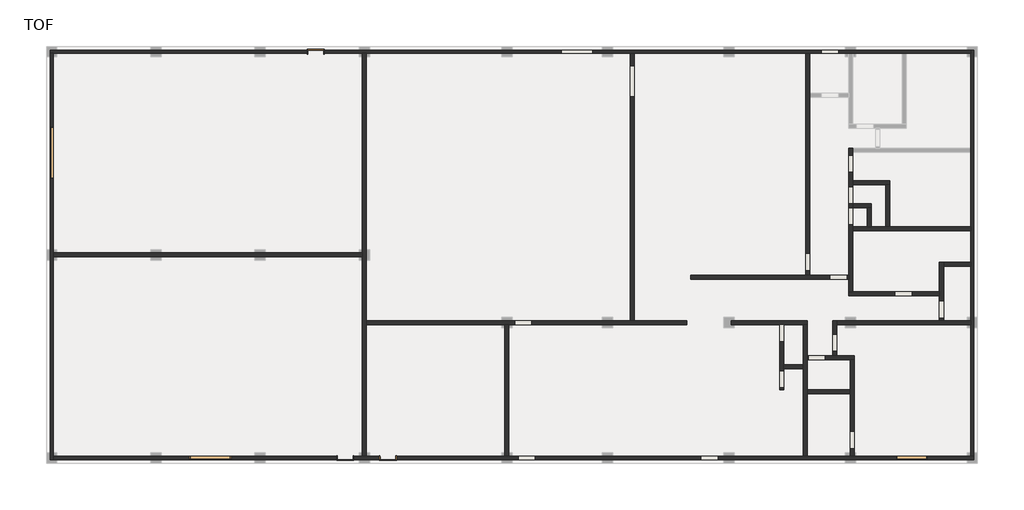
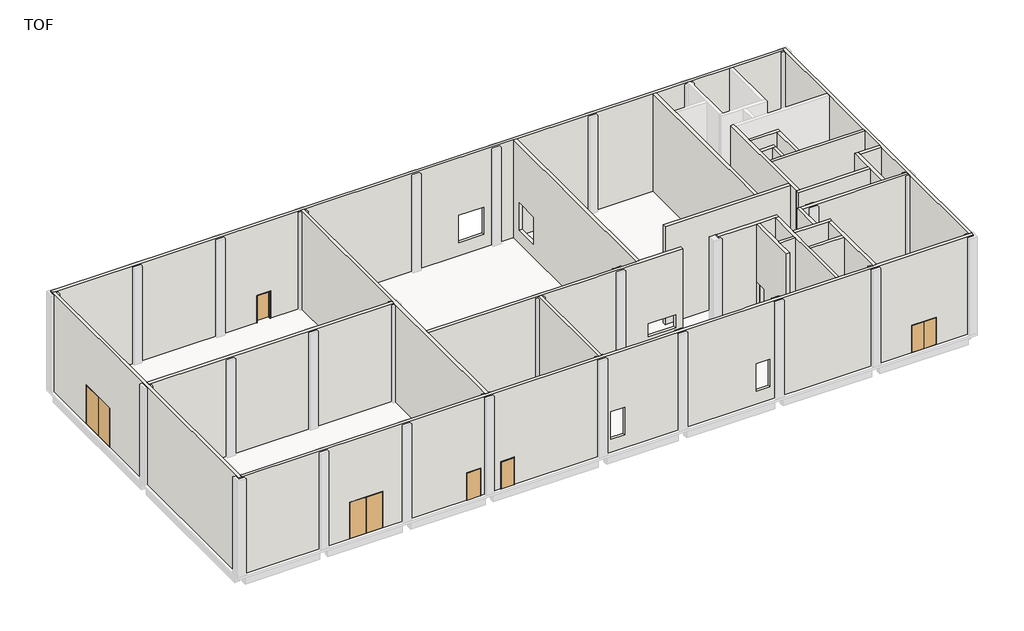
# One storey, part 1 of 2: 29 walls, 6 doors.
"""IFC4 building model written with IfcOpenShell, lengths in millimetres."""

import ifcopenshell
import ifcopenshell.guid

model = None  # the IFC model being written
_history = None  # IfcOwnerHistory: only IFC2X3 demands one
_inside = {}  # id of a spatial element -> (the spatial element, [elements in it])
_under = {}  # id of a project, library or spatial element -> (it, [spatial elements below it])
_declared = {}  # id of a project -> (the project, [libraries it declares])
_typed = {}  # id of a type object -> (the type object, [elements of that type])
_made_of = {}  # id of a material, layer set ... -> (it, [elements and type objects made of it])


def new_model(schema):
    """Start an empty IFC model of exactly this schema.

    Asked for "IFC4X3", IfcOpenShell would pick the latest addendum, in which some entities
    have other attributes; the version numbers below select the first issue.
    IFC2X3 requires an IfcOwnerHistory on every rooted entity: one is made here for all.
    """
    global model, _history
    if schema == "IFC4X3":
        model = ifcopenshell.file(schema_version=(4, 3, 0, 0))
    else:
        model = ifcopenshell.file(schema=schema)
    _inside.clear()
    _under.clear()
    _declared.clear()
    _typed.clear()
    _made_of.clear()
    _history = None
    if model.schema == "IFC2X3":
        org = make("IfcOrganization", Name="unknown")
        user = make(
            "IfcPersonAndOrganization",
            ThePerson=make("IfcPerson", FamilyName="unknown"),
            TheOrganization=org,
        )
        app = make(
            "IfcApplication",
            ApplicationDeveloper=org,
            Version="unknown",
            ApplicationFullName="unknown",
            ApplicationIdentifier="unknown",
        )
        _history = make(
            "IfcOwnerHistory",
            OwningUser=user,
            OwningApplication=app,
            ChangeAction="ADDED",
            CreationDate=0,
        )
    return model


def make(cls, **values):
    """One entity of the class cls with the attributes given. An attribute that is None is left unset."""
    return model.create_entity(
        cls, **{name: value for name, value in values.items() if value is not None}
    )


def rooted(cls, **values):
    """An entity with a GlobalId (a new one), such as an element, a storey or a relation."""
    return make(cls, GlobalId=ifcopenshell.guid.new(), OwnerHistory=_history, **values)


def si_unit(unit_type, name, prefix=None):
    """IfcSIUnit, for example si_unit("LENGTHUNIT", "METRE", prefix="MILLI")."""
    return make("IfcSIUnit", UnitType=unit_type, Prefix=prefix, Name=name)


def assignment(units):
    """IfcUnitAssignment: the units of a project."""
    return None if units is None else make("IfcUnitAssignment", Units=units)


def point(xyz):
    """IfcCartesianPoint."""
    return None if xyz is None else make("IfcCartesianPoint", Coordinates=xyz)


def direction(xyz):
    """IfcDirection."""
    return None if xyz is None else make("IfcDirection", DirectionRatios=xyz)


def frame(location, z_axis=None, x_axis=None):
    """IfcAxis2Placement3D, a coordinate frame: its origin and axes. An axis left out is left unset."""
    return make(
        "IfcAxis2Placement3D",
        Location=point(location),
        Axis=direction(z_axis),
        RefDirection=direction(x_axis),
    )


def origin():
    """The frame at (0, 0, 0) with its axes left unset."""
    return frame((0.0, 0.0, 0.0))


def origin_with_axes():
    """The frame at (0, 0, 0) with the z axis (0, 0, 1) and the x axis (1, 0, 0) written out."""
    return frame((0.0, 0.0, 0.0), z_axis=(0.0, 0.0, 1.0), x_axis=(1.0, 0.0, 0.0))


def place(relative_to, where):
    """IfcLocalPlacement: puts the frame where relative to a parent placement (None: the world)."""
    return make(
        "IfcLocalPlacement", PlacementRelTo=relative_to, RelativePlacement=where
    )


def context(
    kind, dimensions, precision=None, world=None, true_north=None, identifier=None
):
    """IfcGeometricRepresentationContext, for example the 3D "Model" context."""
    return make(
        "IfcGeometricRepresentationContext",
        ContextIdentifier=identifier,
        ContextType=kind,
        CoordinateSpaceDimension=dimensions,
        Precision=precision,
        WorldCoordinateSystem=world,
        TrueNorth=true_north,
    )


def project(units=None, contexts=None):
    """IfcProject with its units and contexts."""
    return rooted(
        "IfcProject",
        Name="project",
        RepresentationContexts=contexts,
        UnitsInContext=assignment(units),
    )


def spatial(cls, under=None, at=None, **own):
    """A site, building, storey or space (cls), placed at a placement, below another one or the project."""
    s = rooted(cls, ObjectPlacement=at, **own)
    if under is not None:
        _under.setdefault(under.id(), (under, []))[1].append(s)
    return s


def polyline(points):
    """IfcPolyline through the points."""
    return make("IfcPolyline", Points=[point(p) for p in points])


def outline(outer, holes=None, kind="AREA"):
    """IfcArbitraryClosedProfileDef: a profile drawn as a closed curve; with holes, ...WithVoids."""
    if holes is None:
        return make("IfcArbitraryClosedProfileDef", ProfileType=kind, OuterCurve=outer)
    return make(
        "IfcArbitraryProfileDefWithVoids",
        ProfileType=kind,
        OuterCurve=outer,
        InnerCurves=holes,
    )


def extrude(swept, where, along, depth):
    """IfcExtrudedAreaSolid: the profile swept, set in the frame where, extruded along a direction by depth."""
    return make(
        "IfcExtrudedAreaSolid",
        SweptArea=swept,
        Position=where,
        ExtrudedDirection=direction(along),
        Depth=depth,
    )


def faces_of(points, faces, orient=None, outer=None):
    """IfcFace entities. A face is a list of loops; a loop is a list of indices into points, from 0.

    orient and outer hold one flag for each loop. By default every Orientation is true, the
    first loop of a face is its IfcFaceOuterBound and the others are IfcFaceBound.
    """
    made = []
    for i, loops in enumerate(faces):
        bounds = []
        for j, loop in enumerate(loops):
            is_outer = j == 0 if outer is None else outer[i][j]
            bounds.append(
                make(
                    "IfcFaceOuterBound" if is_outer else "IfcFaceBound",
                    Bound=make("IfcPolyLoop", Polygon=[points[k] for k in loop]),
                    Orientation=True if orient is None else orient[i][j],
                )
            )
        made.append(make("IfcFace", Bounds=bounds))
    return made


def faceted_brep(points, faces, orient=None, outer=None, voids=None):
    """IfcFacetedBrep: a solid bounded by flat faces; with voids (closed shells), ...WithVoids."""
    shared = [point(p) for p in points]
    hull = make("IfcClosedShell", CfsFaces=faces_of(shared, faces, orient, outer))
    if voids is None:
        return make("IfcFacetedBrep", Outer=hull)
    return make(
        "IfcFacetedBrepWithVoids",
        Outer=hull,
        Voids=[
            make(cls, CfsFaces=faces_of(shared, fs, o, b)) for cls, fs, o, b in voids
        ],
    )


def shape(context_of_items, identifier, shape_type, items):
    """IfcShapeRepresentation: the items that make up one representation, for example the "Body"."""
    return make(
        "IfcShapeRepresentation",
        ContextOfItems=context_of_items,
        RepresentationIdentifier=identifier,
        RepresentationType=shape_type,
        Items=items,
    )


def source(mapping_origin, context_of_items, identifier, shape_type, items):
    """IfcRepresentationMap: a shape defined once, which mapped items show again and again."""
    return make(
        "IfcRepresentationMap",
        MappingOrigin=mapping_origin,
        MappedRepresentation=shape(context_of_items, identifier, shape_type, items),
    )


def transform(
    local_origin,
    x_axis=None,
    y_axis=None,
    z_axis=None,
    scale=None,
    scale2=None,
    scale3=None,
    uniform=True,
):
    """IfcCartesianTransformationOperator3D, or its non-uniform kind. x_axis, y_axis, z_axis: its Axis1, 2, 3."""
    if uniform:
        return make(
            "IfcCartesianTransformationOperator3D",
            Axis1=direction(x_axis),
            Axis2=direction(y_axis),
            LocalOrigin=point(local_origin),
            Scale=scale,
            Axis3=direction(z_axis),
        )
    return make(
        "IfcCartesianTransformationOperator3DnonUniform",
        Axis1=direction(x_axis),
        Axis2=direction(y_axis),
        LocalOrigin=point(local_origin),
        Scale=scale,
        Axis3=direction(z_axis),
        Scale2=scale2,
        Scale3=scale3,
    )


def mapped(mapping_source, mapping_target):
    """IfcMappedItem: shows the shape of a source again, moved by a transform."""
    return make(
        "IfcMappedItem", MappingSource=mapping_source, MappingTarget=mapping_target
    )


def made_of(thing, what):
    """Note that an element or type object is made of a material, layer set ...; save() writes the relation."""
    if what is not None:
        _made_of.setdefault(what.id(), (what, []))[1].append(thing)
    return thing


def element(
    cls,
    number,
    at=None,
    inside=None,
    cuts=None,
    type_object=None,
    material=None,
    context=None,
    identifier="Body",
    shape_type=None,
    held_by="IfcProductDefinitionShape",
    body=None,
    shapes=None,
    **own,
):
    """One element of the class cls, such as IfcWall. Its Tag is "e" and its number.

    at: its placement. inside: the storey or other place that contains it. cuts: it is an
    opening in that element (IfcRelVoidsElement). A single representation is given by context,
    identifier, shape_type and body (its items); several are given by shapes. held_by: the class
    of the entity that holds the representations. save() writes the other relations.
    """
    e = rooted(cls, Tag="e%d" % number, ObjectPlacement=at, **own)
    if body is not None:
        shapes = [shape(context, identifier, shape_type, body)]
    if shapes is not None:
        e.Representation = make(held_by, Representations=shapes)
    if inside is not None:
        _inside.setdefault(inside.id(), (inside, []))[1].append(e)
    if cuts is not None:
        rooted(
            "IfcRelVoidsElement", RelatingBuildingElement=cuts, RelatedOpeningElement=e
        )
    if type_object is not None:
        _typed.setdefault(type_object.id(), (type_object, []))[1].append(e)
    return made_of(e, material)


def aggregate(whole, parts):
    """IfcRelAggregates: a whole, such as a stair, and the parts it consists of."""
    return rooted("IfcRelAggregates", RelatingObject=whole, RelatedObjects=parts)


def save(model, path):
    """Write the relations noted so far, then the file.

    IfcRelAggregates (storeys below a building ...), IfcRelContainedInSpatialStructure (elements
    in a storey), IfcRelDefinesByType, IfcRelAssociatesMaterial and IfcRelDeclares: one each for
    every whole, place, type object, material and project.
    """
    for whole, parts in _under.values():
        aggregate(whole, parts)
    for where, things in _inside.values():
        rooted(
            "IfcRelContainedInSpatialStructure",
            RelatedElements=things,
            RelatingStructure=where,
        )
    for kind, things in _typed.values():
        rooted("IfcRelDefinesByType", RelatedObjects=things, RelatingType=kind)
    for what, things in _made_of.values():
        rooted("IfcRelAssociatesMaterial", RelatedObjects=things, RelatingMaterial=what)
    for by, libraries in _declared.values():
        rooted("IfcRelDeclares", RelatingContext=by, RelatedDefinitions=libraries)
    model.write(path)


def double_door_steel_22a565f0(model_context):
    return source(origin(), model_context, "Body", "SolidModel", [
        extrude(outline(polyline([(880.0, 60.0), (0.0, 60.0), (0.0, 100.0), (880.0, 100.0), (880.0, 60.0)])), frame((0.0, 0.0, 20.0), z_axis=(0.0, 0.0, 1.0), x_axis=(1.0, 0.0, 0.0)), (0.0, 0.0, 1.0), 2060.0),
        extrude(outline(polyline([(0.0, 60.0), (-880.0, 60.0), (-880.0, 100.0), (0.0, 100.0), (0.0, 60.0)])), frame((0.0, 0.0, 20.0), z_axis=(0.0, 0.0, 1.0), x_axis=(1.0, 0.0, 0.0)), (0.0, 0.0, 1.0), 2060.0),
        faceted_brep([(900.0, -100.0, 2100.0), (900.0, 100.0, 2100.0), (-900.0, 100.0, 2100.0), (-900.0, -100.0, 2100.0), (865.0, 60.0, 2065.0), (865.0, -100.0, 2065.0), (-865.0, -100.0, 2065.0), (-865.0, 60.0, 2065.0), (880.0, 100.0, 2080.0), (880.0, 60.0, 2080.0), (-880.0, 60.0, 2080.0), (-880.0, 100.0, 2080.0), (-900.0, 100.0, 0.0), (-900.0, -100.0, 0.0), (-865.0, -100.0, 35.0), (-865.0, 60.0, 35.0), (-880.0, 60.0, 20.0), (-880.0, 100.0, 20.0), (900.0, 100.0, 0.0), (880.0, 100.0, 20.0), (900.0, -100.0, 0.0), (865.0, -100.0, 35.0), (865.0, 60.0, 35.0), (880.0, 60.0, 20.0)], [[[0, 1, 2, 3]], [[4, 5, 6, 7]], [[8, 9, 10, 11]], [[3, 2, 12, 13]], [[7, 6, 14, 15]], [[11, 10, 16, 17]], [[18, 12, 2, 1], [8, 11, 17, 19]], [[13, 12, 18, 20]], [[0, 3, 13, 20], [21, 14, 6, 5]], [[15, 14, 21, 22]], [[23, 16, 10, 9], [4, 7, 15, 22]], [[17, 16, 23, 19]], [[20, 18, 1, 0]], [[22, 21, 5, 4]], [[19, 23, 9, 8]]]),
    ])


def double_door_steel_3c26782d(model_context):
    return source(origin(), model_context, "Body", "SolidModel", [
        extrude(outline(polyline([(1180.0, 60.0), (0.0, 60.0), (0.0, 100.0), (1180.0, 100.0), (1180.0, 60.0)])), frame((0.0, 0.0, 20.0), z_axis=(0.0, 0.0, 1.0), x_axis=(1.0, 0.0, 0.0)), (0.0, 0.0, 1.0), 2760.0),
        extrude(outline(polyline([(0.0, 60.0), (-1180.0, 60.0), (-1180.0, 100.0), (0.0, 100.0), (0.0, 60.0)])), frame((0.0, 0.0, 20.0), z_axis=(0.0, 0.0, 1.0), x_axis=(1.0, 0.0, 0.0)), (0.0, 0.0, 1.0), 2760.0),
        faceted_brep([(1200.0, -100.0, 2800.0), (1200.0, 100.0, 2800.0), (-1200.0, 100.0, 2800.0), (-1200.0, -100.0, 2800.0), (1165.0, 60.0, 2765.0), (1165.0, -100.0, 2765.0), (-1165.0, -100.0, 2765.0), (-1165.0, 60.0, 2765.0), (1180.0, 100.0, 2780.0), (1180.0, 60.0, 2780.0), (-1180.0, 60.0, 2780.0), (-1180.0, 100.0, 2780.0), (-1200.0, 100.0, 0.0), (-1200.0, -100.0, 0.0), (-1165.0, -100.0, 35.0), (-1165.0, 60.0, 35.0), (-1180.0, 60.0, 20.0), (-1180.0, 100.0, 20.0), (1200.0, 100.0, 0.0), (1180.0, 100.0, 20.0), (1200.0, -100.0, 0.0), (1165.0, -100.0, 35.0), (1165.0, 60.0, 35.0), (1180.0, 60.0, 20.0)], [[[0, 1, 2, 3]], [[4, 5, 6, 7]], [[8, 9, 10, 11]], [[3, 2, 12, 13]], [[7, 6, 14, 15]], [[11, 10, 16, 17]], [[18, 12, 2, 1], [8, 11, 17, 19]], [[13, 12, 18, 20]], [[0, 3, 13, 20], [21, 14, 6, 5]], [[15, 14, 21, 22]], [[23, 16, 10, 9], [4, 7, 15, 22]], [[17, 16, 23, 19]], [[20, 18, 1, 0]], [[22, 21, 5, 4]], [[19, 23, 9, 8]]]),
    ])


def double_door_steel_ab4802d0(model_context):
    return source(origin(), model_context, "Body", "SolidModel", [
        extrude(outline(polyline([(1480.0, 60.0), (0.0, 60.0), (0.0, 100.0), (1480.0, 100.0), (1480.0, 60.0)])), frame((0.0, 0.0, 20.0), z_axis=(0.0, 0.0, 1.0), x_axis=(1.0, 0.0, 0.0)), (0.0, 0.0, 1.0), 2960.0),
        extrude(outline(polyline([(0.0, 60.0), (-1480.0, 60.0), (-1480.0, 100.0), (0.0, 100.0), (0.0, 60.0)])), frame((0.0, 0.0, 20.0), z_axis=(0.0, 0.0, 1.0), x_axis=(1.0, 0.0, 0.0)), (0.0, 0.0, 1.0), 2960.0),
        faceted_brep([(1500.0, -100.0, 3000.0), (1500.0, 100.0, 3000.0), (-1500.0, 100.0, 3000.0), (-1500.0, -100.0, 3000.0), (1465.0, 60.0, 2965.0), (1465.0, -100.0, 2965.0), (-1465.0, -100.0, 2965.0), (-1465.0, 60.0, 2965.0), (1480.0, 100.0, 2980.0), (1480.0, 60.0, 2980.0), (-1480.0, 60.0, 2980.0), (-1480.0, 100.0, 2980.0), (-1500.0, 100.0, 0.0), (-1500.0, -100.0, 0.0), (-1465.0, -100.0, 35.0), (-1465.0, 60.0, 35.0), (-1480.0, 60.0, 20.0), (-1480.0, 100.0, 20.0), (1500.0, 100.0, 0.0), (1480.0, 100.0, 20.0), (1500.0, -100.0, 0.0), (1465.0, -100.0, 35.0), (1465.0, 60.0, 35.0), (1480.0, 60.0, 20.0)], [[[0, 1, 2, 3]], [[4, 5, 6, 7]], [[8, 9, 10, 11]], [[3, 2, 12, 13]], [[7, 6, 14, 15]], [[11, 10, 16, 17]], [[18, 12, 2, 1], [8, 11, 17, 19]], [[13, 12, 18, 20]], [[0, 3, 13, 20], [21, 14, 6, 5]], [[15, 14, 21, 22]], [[23, 16, 10, 9], [4, 7, 15, 22]], [[17, 16, 23, 19]], [[20, 18, 1, 0]], [[22, 21, 5, 4]], [[19, 23, 9, 8]]]),
    ])


def single_door_steel_02f153ad(model_context):
    return source(origin(), model_context, "Body", "SolidModel", [
        extrude(outline(polyline([(470.0, -130.0), (-470.0, -130.0), (-470.0, -95.0), (470.0, -95.0), (470.0, -130.0)])), origin_with_axes(), (0.0, 0.0, 1.0), 2070.0),
        faceted_brep([(470.0, -130.0, 0.0), (470.0, -95.0, 0.0), (450.0, -95.0, 0.0), (450.0, 95.0, 0.0), (470.0, 95.0, 0.0), (470.0, 130.0, 0.0), (500.0, 130.0, 0.0), (500.0, -130.0, 0.0), (500.0, -130.0, 2100.0), (-500.0, -130.0, 2100.0), (-500.0, -130.0, 0.0), (-470.0, -130.0, 0.0), (-470.0, -130.0, 2070.0), (470.0, -130.0, 2070.0), (500.0, 130.0, 2100.0), (470.0, 130.0, 2070.0), (-470.0, 130.0, 2070.0), (-470.0, 130.0, 0.0), (-500.0, 130.0, 0.0), (-500.0, 130.0, 2100.0), (470.0, 95.0, 2070.0), (450.0, 95.0, 2050.0), (-450.0, 95.0, 2050.0), (-450.0, 95.0, 0.0), (-470.0, 95.0, 0.0), (-470.0, 95.0, 2070.0), (450.0, -95.0, 2050.0), (470.0, -95.0, 2070.0), (-470.0, -95.0, 2070.0), (-470.0, -95.0, 0.0), (-450.0, -95.0, 0.0), (-450.0, -95.0, 2050.0)], [[[0, 1, 2, 3, 4, 5, 6, 7]], [[7, 8, 9, 10, 11, 12, 13, 0]], [[6, 14, 8, 7]], [[5, 15, 16, 17, 18, 19, 14, 6]], [[4, 20, 15, 5]], [[3, 21, 22, 23, 24, 25, 20, 4]], [[2, 26, 21, 3]], [[1, 27, 28, 29, 30, 31, 26, 2]], [[0, 13, 27, 1]], [[12, 11, 29, 28]], [[11, 10, 18, 17, 24, 23, 30, 29]], [[19, 18, 10, 9]], [[25, 24, 17, 16]], [[31, 30, 23, 22]], [[14, 19, 9, 8]], [[20, 25, 16, 15]], [[26, 31, 22, 21]], [[13, 12, 28, 27]]]),
    ])


def single_door_steel_4a6c7de9(model_context):
    return source(origin(), model_context, "Body", "SolidModel", [
        extrude(outline(polyline([(470.0, 130.0), (470.0, 95.0), (-470.0, 95.0), (-470.0, 130.0), (470.0, 130.0)])), origin_with_axes(), (0.0, 0.0, 1.0), 2070.0),
        faceted_brep([(470.0, 130.0, 0.0), (500.0, 130.0, 0.0), (500.0, -130.0, 0.0), (470.0, -130.0, 0.0), (470.0, -95.0, 0.0), (450.0, -95.0, 0.0), (450.0, 95.0, 0.0), (470.0, 95.0, 0.0), (470.0, 130.0, 2070.0), (-470.0, 130.0, 2070.0), (-470.0, 130.0, 0.0), (-500.0, 130.0, 0.0), (-500.0, 130.0, 2100.0), (500.0, 130.0, 2100.0), (500.0, -130.0, 2100.0), (-500.0, -130.0, 2100.0), (-500.0, -130.0, 0.0), (-470.0, -130.0, 0.0), (-470.0, -130.0, 2070.0), (470.0, -130.0, 2070.0), (470.0, -95.0, 2070.0), (-470.0, -95.0, 2070.0), (-470.0, -95.0, 0.0), (-450.0, -95.0, 0.0), (-450.0, -95.0, 2050.0), (450.0, -95.0, 2050.0), (450.0, 95.0, 2050.0), (-450.0, 95.0, 2050.0), (-450.0, 95.0, 0.0), (-470.0, 95.0, 0.0), (-470.0, 95.0, 2070.0), (470.0, 95.0, 2070.0)], [[[0, 1, 2, 3, 4, 5, 6, 7]], [[1, 0, 8, 9, 10, 11, 12, 13]], [[2, 1, 13, 14]], [[3, 2, 14, 15, 16, 17, 18, 19]], [[4, 3, 19, 20]], [[5, 4, 20, 21, 22, 23, 24, 25]], [[6, 5, 25, 26]], [[7, 6, 26, 27, 28, 29, 30, 31]], [[0, 7, 31, 8]], [[9, 30, 29, 10]], [[10, 29, 28, 23, 22, 17, 16, 11]], [[15, 12, 11, 16]], [[21, 18, 17, 22]], [[27, 24, 23, 28]], [[14, 13, 12, 15]], [[20, 19, 18, 21]], [[26, 25, 24, 27]], [[8, 31, 30, 9]]]),
    ])


model = new_model("IFC4")

# Units and contexts
model_context = context("Model", 3, world=origin())
ifc_project = project(units=[si_unit("LENGTHUNIT", "METRE", prefix="MILLI")], contexts=[model_context])

# Site, building, storey
site = spatial("IfcSite", under=ifc_project)
building = spatial("IfcBuilding", under=site)
storey = spatial("IfcBuildingStorey", under=building, Name="TOF", Elevation=149.9618634)

# Doors
placement = place(None, origin())
double_door_steel_shape = double_door_steel_22a565f0(model_context)
element("IfcDoor", 1, ObjectType="Double Door_Steel", at=placement, inside=storey, context=model_context, shape_type="MappedRepresentation", body=[
    mapped(double_door_steel_shape, transform((49525.0, 499.5208589, 149.9618634), x_axis=(-1.0, 0.0, 0.0), y_axis=(0.0, -1.0, 0.0), z_axis=(0.0, 0.0, 1.0))),
])
double_door_steel_2_shape = double_door_steel_3c26782d(model_context)
element("IfcDoor", 2, ObjectType="Double Door_Steel", at=placement, inside=storey, context=model_context, shape_type="MappedRepresentation", body=[
    mapped(double_door_steel_2_shape, transform((9125.0, 499.5208589, 149.9618634), x_axis=(-1.0, 0.0, 0.0), y_axis=(0.0, -1.0, 0.0), z_axis=(0.0, 0.0, 1.0))),
])
double_door_steel_3_shape = double_door_steel_ab4802d0(model_context)
element("IfcDoor", 3, ObjectType="Double Door_Steel", at=placement, inside=storey, context=model_context, shape_type="MappedRepresentation", body=[
    mapped(double_door_steel_3_shape, transform((0.0, 18074.5208589, 149.9618634), x_axis=(0.0, 1.0, 0.0), y_axis=(-1.0, 0.0, 0.0), z_axis=(0.0, 0.0, 1.0))),
])
single_door_steel_shape = single_door_steel_02f153ad(model_context)
element("IfcDoor", 4, ObjectType="Single Door_Steel", at=placement, inside=storey, context=model_context, shape_type="MappedRepresentation", body=[
    mapped(single_door_steel_shape, transform((15200.0, 23899.5208589, 149.9618634), x_axis=(-1.0, 0.0, 0.0), y_axis=(0.0, -1.0, 0.0), z_axis=(0.0, 0.0, 1.0))),
])
element("IfcDoor", 5, ObjectType="Single Door_Steel", at=placement, inside=storey, context=model_context, shape_type="MappedRepresentation", body=[
    mapped(single_door_steel_shape, transform((19350.0, 499.5208589, 149.9618634), x_axis=(1.0, 0.0, 0.0), y_axis=(0.0, 1.0, 0.0), z_axis=(0.0, 0.0, 1.0))),
])
single_door_steel_2_shape = single_door_steel_4a6c7de9(model_context)
element("IfcDoor", 6, ObjectType="Single Door_Steel", at=placement, inside=storey, context=model_context, shape_type="MappedRepresentation", body=[
    mapped(single_door_steel_2_shape, transform((16900.0, 499.5208589, 149.9618634), x_axis=(-1.0, 0.0, 0.0), y_axis=(0.0, -1.0, 0.0), z_axis=(0.0, 0.0, 1.0))),
])

# Walls
element("IfcWall", 7, at=placement, inside=storey, context=model_context, shape_type="Brep", body=[
    faceted_brep([(52900.0, 23799.5208589, 7649.9618634), (49197.0, 23799.5208589, 7649.9618634), (48963.0, 23799.5208589, 7649.9618634), (46117.0, 23799.5208589, 7649.9618634), (45883.0, 23799.5208589, 7649.9618634), (43647.0, 23799.5208589, 7649.9618634), (43413.0, 23799.5208589, 7649.9618634), (33537.0, 23799.5208589, 7649.9618634), (33303.0, 23799.5208589, 7649.9618634), (18112.0, 23799.5208589, 7649.9618634), (17878.0, 23799.5208589, 7649.9618634), (100.0, 23799.5208589, 7649.9618634), (-100.0, 23799.5208589, 7649.9618634), (-100.0, 23799.5208589, 149.9618634), (100.0, 23799.5208589, 149.9618634), (14700.0, 23799.5208589, 149.9618634), (14700.0, 23799.5208589, 2249.9618634), (15700.0, 23799.5208589, 2249.9618634), (15700.0, 23799.5208589, 149.9618634), (17878.0, 23799.5208589, 149.9618634), (18112.0, 23799.5208589, 149.9618634), (33303.0, 23799.5208589, 149.9618634), (33537.0, 23799.5208589, 149.9618634), (43413.0, 23799.5208589, 149.9618634), (43647.0, 23799.5208589, 149.9618634), (45883.0, 23799.5208589, 149.9618634), (46117.0, 23799.5208589, 149.9618634), (48963.0, 23799.5208589, 149.9618634), (49197.0, 23799.5208589, 149.9618634), (52900.0, 23799.5208589, 149.9618634), (31150.0, 23799.5208589, 1149.9618634), (29350.0, 23799.5208589, 1149.9618634), (29350.0, 23799.5208589, 3249.9618634), (31150.0, 23799.5208589, 3249.9618634), (44300.0, 23799.5208589, 1149.9618634), (44300.0, 23799.5208589, 3249.9618634), (45300.0, 23799.5208589, 3249.9618634), (45300.0, 23799.5208589, 1149.9618634), (-100.0, 23999.5208589, 7649.9618634), (52900.0, 23999.5208589, 7649.9618634), (52900.0, 23999.5208589, 149.9618634), (15700.0, 23999.5208589, 149.9618634), (15700.0, 23999.5208589, 2249.9618634), (14700.0, 23999.5208589, 2249.9618634), (14700.0, 23999.5208589, 149.9618634), (-100.0, 23999.5208589, 149.9618634), (31150.0, 23999.5208589, 1149.9618634), (31150.0, 23999.5208589, 3249.9618634), (29350.0, 23999.5208589, 3249.9618634), (29350.0, 23999.5208589, 1149.9618634), (44300.0, 23999.5208589, 1149.9618634), (45300.0, 23999.5208589, 1149.9618634), (45300.0, 23999.5208589, 3249.9618634), (44300.0, 23999.5208589, 3249.9618634)], [[[0, 1, 2, 3, 4, 5, 6, 7, 8, 9, 10, 11, 12, 13, 14, 15, 16, 17, 18, 19, 20, 21, 22, 23, 24, 25, 26, 27, 28, 29], [30, 31, 32, 33], [34, 35, 36, 37]], [[38, 39, 40, 41, 42, 43, 44, 45], [46, 47, 48, 49], [50, 51, 52, 53]], [[13, 45, 44, 15, 14]], [[40, 29, 28, 27, 26, 25, 24, 23, 22, 21, 20, 19, 18, 41]], [[12, 11, 10, 9, 8, 7, 6, 5, 4, 3, 2, 1, 0, 39, 38]], [[13, 12, 38, 45]], [[0, 29, 40, 39]], [[47, 46, 30, 33]], [[48, 47, 33, 32]], [[49, 48, 32, 31]], [[46, 49, 31, 30]], [[35, 34, 50, 53]], [[36, 35, 53, 52]], [[37, 36, 52, 51]], [[34, 37, 51, 50]], [[43, 16, 15, 44]], [[16, 43, 42, 17]], [[17, 42, 41, 18]]]),
])
element("IfcWall", 8, at=placement, inside=storey, context=model_context, shape_type="Brep", body=[
    faceted_brep([(100.0, 23799.5208589, 7649.9618634), (100.0, 12316.5208589, 7649.9618634), (100.0, 12082.5208589, 7649.9618634), (100.0, 599.5208589, 7649.9618634), (100.0, 399.5208589, 7649.9618634), (100.0, 399.5208589, 149.9618634), (100.0, 599.5208589, 149.9618634), (100.0, 12082.5208589, 149.9618634), (100.0, 12316.5208589, 149.9618634), (100.0, 16574.5208589, 149.9618634), (100.0, 16574.5208589, 3149.9618634), (100.0, 19574.5208589, 3149.9618634), (100.0, 19574.5208589, 149.9618634), (100.0, 23799.5208589, 149.9618634), (-100.0, 399.5208589, 7649.9618634), (-100.0, 23799.5208589, 7649.9618634), (-100.0, 23799.5208589, 149.9618634), (-100.0, 19574.5208589, 149.9618634), (-100.0, 19574.5208589, 3149.9618634), (-100.0, 16574.5208589, 3149.9618634), (-100.0, 16574.5208589, 149.9618634), (-100.0, 399.5208589, 149.9618634)], [[[0, 1, 2, 3, 4, 5, 6, 7, 8, 9, 10, 11, 12, 13]], [[14, 15, 16, 17, 18, 19, 20, 21]], [[5, 21, 20, 9, 8, 7, 6]], [[16, 13, 12, 17]], [[4, 3, 2, 1, 0, 15, 14]], [[5, 4, 14, 21]], [[0, 13, 16, 15]], [[11, 18, 17, 12]], [[18, 11, 10, 19]], [[19, 10, 9, 20]]]),
])
element("IfcWall", 9, at=placement, inside=storey, context=model_context, shape_type="Brep", body=[
    faceted_brep([(100.0, 599.5208589, 7649.9618634), (17878.0, 599.5208589, 7649.9618634), (18112.0, 599.5208589, 7649.9618634), (26078.0, 599.5208589, 7649.9618634), (26312.0, 599.5208589, 7649.9618634), (28628.0, 599.5208589, 7649.9618634), (28862.0, 599.5208589, 7649.9618634), (31883.0, 599.5208589, 7649.9618634), (32117.0, 599.5208589, 7649.9618634), (36553.0, 599.5208589, 7649.9618634), (36787.0, 599.5208589, 7649.9618634), (38888.0, 599.5208589, 7649.9618634), (39122.0, 599.5208589, 7649.9618634), (43263.0, 599.5208589, 7649.9618634), (43497.0, 599.5208589, 7649.9618634), (45963.0, 599.5208589, 7649.9618634), (46197.0, 599.5208589, 7649.9618634), (52900.0, 599.5208589, 7649.9618634), (53100.0, 599.5208589, 7649.9618634), (53100.0, 599.5208589, 149.9618634), (52900.0, 599.5208589, 149.9618634), (50425.0, 599.5208589, 149.9618634), (50425.0, 599.5208589, 2249.9618634), (48625.0, 599.5208589, 2249.9618634), (48625.0, 599.5208589, 149.9618634), (46197.0, 599.5208589, 149.9618634), (45963.0, 599.5208589, 149.9618634), (43497.0, 599.5208589, 149.9618634), (43263.0, 599.5208589, 149.9618634), (26312.0, 599.5208589, 149.9618634), (26078.0, 599.5208589, 149.9618634), (19850.0, 599.5208589, 149.9618634), (19850.0, 599.5208589, 2249.9618634), (18850.0, 599.5208589, 2249.9618634), (18850.0, 599.5208589, 149.9618634), (18112.0, 599.5208589, 149.9618634), (17878.0, 599.5208589, 149.9618634), (17400.0, 599.5208589, 149.9618634), (17400.0, 599.5208589, 2249.9618634), (16400.0, 599.5208589, 2249.9618634), (16400.0, 599.5208589, 149.9618634), (10325.0, 599.5208589, 149.9618634), (10325.0, 599.5208589, 2949.9618634), (7925.0, 599.5208589, 2949.9618634), (7925.0, 599.5208589, 149.9618634), (100.0, 599.5208589, 149.9618634), (27850.0, 599.5208589, 1149.9618634), (27850.0, 599.5208589, 3249.9618634), (26850.0, 599.5208589, 3249.9618634), (26850.0, 599.5208589, 1149.9618634), (37375.0, 599.5208589, 1149.9618634), (38375.0, 599.5208589, 1149.9618634), (38375.0, 599.5208589, 3249.9618634), (37375.0, 599.5208589, 3249.9618634), (53100.0, 399.5208589, 7649.9618634), (100.0, 399.5208589, 7649.9618634), (100.0, 399.5208589, 149.9618634), (7925.0, 399.5208589, 149.9618634), (7925.0, 399.5208589, 2949.9618634), (10325.0, 399.5208589, 2949.9618634), (10325.0, 399.5208589, 149.9618634), (16400.0, 399.5208589, 149.9618634), (16400.0, 399.5208589, 2249.9618634), (17400.0, 399.5208589, 2249.9618634), (17400.0, 399.5208589, 149.9618634), (18850.0, 399.5208589, 149.9618634), (18850.0, 399.5208589, 2249.9618634), (19850.0, 399.5208589, 2249.9618634), (19850.0, 399.5208589, 149.9618634), (48625.0, 399.5208589, 149.9618634), (48625.0, 399.5208589, 2249.9618634), (50425.0, 399.5208589, 2249.9618634), (50425.0, 399.5208589, 149.9618634), (53100.0, 399.5208589, 149.9618634), (27850.0, 399.5208589, 1149.9618634), (26850.0, 399.5208589, 1149.9618634), (26850.0, 399.5208589, 3249.9618634), (27850.0, 399.5208589, 3249.9618634), (37375.0, 399.5208589, 1149.9618634), (37375.0, 399.5208589, 3249.9618634), (38375.0, 399.5208589, 3249.9618634), (38375.0, 399.5208589, 1149.9618634)], [[[0, 1, 2, 3, 4, 5, 6, 7, 8, 9, 10, 11, 12, 13, 14, 15, 16, 17, 18, 19, 20, 21, 22, 23, 24, 25, 26, 27, 28, 29, 30, 31, 32, 33, 34, 35, 36, 37, 38, 39, 40, 41, 42, 43, 44, 45], [46, 47, 48, 49], [50, 51, 52, 53]], [[54, 55, 56, 57, 58, 59, 60, 61, 62, 63, 64, 65, 66, 67, 68, 69, 70, 71, 72, 73], [74, 75, 76, 77], [78, 79, 80, 81]], [[19, 73, 72, 21, 20]], [[56, 45, 44, 57]], [[60, 41, 40, 61]], [[68, 31, 30, 29, 28, 27, 26, 25, 24, 69]], [[34, 65, 64, 37, 36, 35]], [[18, 17, 16, 15, 14, 13, 12, 11, 10, 9, 8, 7, 6, 5, 4, 3, 2, 1, 0, 55, 54]], [[19, 18, 54, 73]], [[0, 45, 56, 55]], [[47, 46, 74, 77]], [[48, 47, 77, 76]], [[49, 48, 76, 75]], [[46, 49, 75, 74]], [[79, 78, 50, 53]], [[80, 79, 53, 52]], [[81, 80, 52, 51]], [[78, 81, 51, 50]], [[43, 58, 57, 44]], [[58, 43, 42, 59]], [[59, 42, 41, 60]], [[67, 32, 31, 68]], [[32, 67, 66, 33]], [[33, 66, 65, 34]], [[39, 62, 61, 40]], [[62, 39, 38, 63]], [[63, 38, 37, 64]], [[23, 70, 69, 24]], [[70, 23, 22, 71]], [[71, 22, 21, 72]]]),
])
element("IfcWall", 10, at=placement, inside=storey, context=model_context, shape_type="Brep", body=[
    faceted_brep([(52900.0, 23999.5208589, 149.9618634), (52900.0, 23799.5208589, 149.9618634), (52900.0, 18336.5208589, 149.9618634), (52900.0, 18102.5208589, 149.9618634), (52900.0, 13836.5208589, 149.9618634), (52900.0, 13602.5208589, 149.9618634), (52900.0, 11786.5208589, 149.9618634), (52900.0, 11552.5208589, 149.9618634), (52900.0, 8411.5208589, 149.9618634), (52900.0, 8177.5208589, 149.9618634), (52900.0, 599.5208589, 149.9618634), (52900.0, 599.5208589, 7649.9618634), (52900.0, 8177.5208589, 7649.9618634), (52900.0, 8411.5208589, 7649.9618634), (52900.0, 11552.5208589, 7649.9618634), (52900.0, 11786.5208589, 7649.9618634), (52900.0, 13602.5208589, 7649.9618634), (52900.0, 13836.5208589, 7649.9618634), (52900.0, 18102.5208589, 7649.9618634), (52900.0, 18336.5208589, 7649.9618634), (52900.0, 23799.5208589, 7649.9618634), (52900.0, 23999.5208589, 7649.9618634), (53100.0, 23999.5208589, 149.9618634), (53100.0, 23999.5208589, 7649.9618634), (53100.0, 599.5208589, 7649.9618634), (53100.0, 599.5208589, 149.9618634)], [[[0, 1, 2, 3, 4, 5, 6, 7, 8, 9, 10, 11, 12, 13, 14, 15, 16, 17, 18, 19, 20, 21]], [[22, 23, 24, 25]], [[10, 9, 8, 7, 6, 5, 4, 3, 2, 1, 0, 22, 25]], [[21, 20, 19, 18, 17, 16, 15, 14, 13, 12, 11, 24, 23]], [[0, 21, 23, 22]], [[11, 10, 25, 24]]]),
])
element("IfcWall", 11, at=placement, inside=storey, context=model_context, shape_type="SweptSolid", body=[
    extrude(outline(polyline([(17878.0, 12082.5208589), (100.0, 12082.5208589), (100.0, 12316.5208589), (17878.0, 12316.5208589), (17878.0, 12082.5208589)])), frame((0.0, 0.0, 149.9618634), z_axis=(0.0, 0.0, 1.0), x_axis=(1.0, 0.0, 0.0)), (0.0, 0.0, 1.0), 7500.0),
])
element("IfcWall", 12, at=placement, inside=storey, context=model_context, shape_type="Brep", body=[
    faceted_brep([(17878.0, 23799.5208589, 149.9618634), (17878.0, 12316.5208589, 149.9618634), (17878.0, 12082.5208589, 149.9618634), (17878.0, 599.5208589, 149.9618634), (17878.0, 599.5208589, 7649.9618634), (17878.0, 12082.5208589, 7649.9618634), (17878.0, 12316.5208589, 7649.9618634), (17878.0, 23799.5208589, 7649.9618634), (18112.0, 23799.5208589, 149.9618634), (18112.0, 23799.5208589, 7649.9618634), (18112.0, 8416.5208589, 7649.9618634), (18112.0, 8182.5208589, 7649.9618634), (18112.0, 599.5208589, 7649.9618634), (18112.0, 599.5208589, 149.9618634), (18112.0, 8182.5208589, 149.9618634), (18112.0, 8416.5208589, 149.9618634)], [[[0, 1, 2, 3, 4, 5, 6, 7]], [[8, 9, 10, 11, 12, 13, 14, 15]], [[3, 2, 1, 0, 8, 15, 14, 13]], [[7, 6, 5, 4, 12, 11, 10, 9]], [[4, 3, 13, 12]], [[0, 7, 9, 8]]]),
])
element("IfcWall", 13, at=placement, inside=storey, context=model_context, shape_type="Brep", body=[
    faceted_brep([(36553.0, 8416.5208589, 149.9618634), (33537.0, 8416.5208589, 149.9618634), (33303.0, 8416.5208589, 149.9618634), (18112.0, 8416.5208589, 149.9618634), (18112.0, 8416.5208589, 7649.9618634), (33303.0, 8416.5208589, 7649.9618634), (33537.0, 8416.5208589, 7649.9618634), (36553.0, 8416.5208589, 7649.9618634), (27650.0, 8416.5208589, 1149.9618634), (27650.0, 8416.5208589, 3249.9618634), (26650.0, 8416.5208589, 3249.9618634), (26650.0, 8416.5208589, 1149.9618634), (36050.0, 8416.5208589, 1749.9618634), (36050.0, 8416.5208589, 2749.9618634), (34050.0, 8416.5208589, 2749.9618634), (34050.0, 8416.5208589, 1749.9618634), (36553.0, 8182.5208589, 149.9618634), (36553.0, 8182.5208589, 7649.9618634), (32117.0, 8182.5208589, 7649.9618634), (31883.0, 8182.5208589, 7649.9618634), (28862.0, 8182.5208589, 7649.9618634), (28628.0, 8182.5208589, 7649.9618634), (26312.0, 8182.5208589, 7649.9618634), (26078.0, 8182.5208589, 7649.9618634), (18112.0, 8182.5208589, 7649.9618634), (18112.0, 8182.5208589, 149.9618634), (26078.0, 8182.5208589, 149.9618634), (26312.0, 8182.5208589, 149.9618634), (27650.0, 8182.5208589, 1149.9618634), (26650.0, 8182.5208589, 1149.9618634), (26650.0, 8182.5208589, 3249.9618634), (27650.0, 8182.5208589, 3249.9618634), (36050.0, 8182.5208589, 1749.9618634), (34050.0, 8182.5208589, 1749.9618634), (34050.0, 8182.5208589, 2749.9618634), (36050.0, 8182.5208589, 2749.9618634)], [[[0, 1, 2, 3, 4, 5, 6, 7], [8, 9, 10, 11], [12, 13, 14, 15]], [[16, 17, 18, 19, 20, 21, 22, 23, 24, 25, 26, 27], [28, 29, 30, 31], [32, 33, 34, 35]], [[3, 2, 1, 0, 16, 27, 26, 25]], [[7, 6, 5, 4, 24, 23, 22, 21, 20, 19, 18, 17]], [[4, 3, 25, 24]], [[0, 7, 17, 16]], [[9, 8, 28, 31]], [[10, 9, 31, 30]], [[11, 10, 30, 29]], [[8, 11, 29, 28]], [[13, 12, 32, 35]], [[14, 13, 35, 34]], [[15, 14, 34, 33]], [[12, 15, 33, 32]]]),
])
element("IfcWall", 14, at=placement, inside=storey, context=model_context, shape_type="SweptSolid", body=[
    extrude(outline(polyline([(23799.5208589, 149.9618634), (8416.5208589, 149.9618634), (8416.5208589, 7649.9618634), (23799.5208589, 7649.9618634), (23799.5208589, 149.9618634)]), holes=[polyline([(23099.5208589, 1149.9618634), (23099.5208589, 3249.9618634), (21299.5208589, 3249.9618634), (21299.5208589, 1149.9618634), (23099.5208589, 1149.9618634)])]), frame((33303.0, 0.0, 0.0), z_axis=(1.0, 0.0, 0.0), x_axis=(0.0, 1.0, 0.0)), (0.0, 0.0, 1.0), 234.0),
])
element("IfcWall", 15, at=placement, inside=storey, context=model_context, shape_type="Brep", body=[
    faceted_brep([(26078.0, 8182.5208589, 149.9618634), (26078.0, 599.5208589, 149.9618634), (26078.0, 599.5208589, 7649.9618634), (26078.0, 8182.5208589, 7649.9618634), (26312.0, 8182.5208589, 149.9618634), (26312.0, 8182.5208589, 7649.9618634), (26312.0, 2859.0208589, 7649.9618634), (26312.0, 2625.0208589, 7649.9618634), (26312.0, 599.5208589, 7649.9618634), (26312.0, 599.5208589, 149.9618634)], [[[0, 1, 2, 3]], [[4, 5, 6, 7, 8, 9]], [[1, 0, 4, 9]], [[3, 2, 8, 7, 6, 5]], [[2, 1, 9, 8]], [[0, 3, 5, 4]]]),
])
element("IfcWall", 16, at=placement, inside=storey, context=model_context, shape_type="Brep", body=[
    faceted_brep([(36787.0, 10802.5208589, 149.9618634), (45883.0, 10802.5208589, 149.9618634), (45883.0, 10802.5208589, 7649.9618634), (36787.0, 10802.5208589, 7649.9618634), (44800.0, 10802.5208589, 1149.9618634), (44800.0, 10802.5208589, 3249.9618634), (45800.0, 10802.5208589, 3249.9618634), (45800.0, 10802.5208589, 1149.9618634), (36787.0, 11036.5208589, 149.9618634), (36787.0, 11036.5208589, 1149.9618634), (36787.0, 11036.5208589, 7649.9618634), (43413.0, 11036.5208589, 7649.9618634), (43647.0, 11036.5208589, 7649.9618634), (45883.0, 11036.5208589, 7649.9618634), (45883.0, 11036.5208589, 149.9618634), (43647.0, 11036.5208589, 149.9618634), (43413.0, 11036.5208589, 149.9618634), (44800.0, 11036.5208589, 1149.9618634), (45800.0, 11036.5208589, 1149.9618634), (45800.0, 11036.5208589, 3249.9618634), (44800.0, 11036.5208589, 3249.9618634)], [[[0, 1, 2, 3], [4, 5, 6, 7]], [[8, 9, 10, 11, 12, 13, 14, 15, 16], [17, 18, 19, 20]], [[1, 0, 8, 16, 15, 14]], [[3, 2, 13, 12, 11, 10]], [[0, 3, 10, 9, 8]], [[2, 1, 14, 13]], [[5, 4, 17, 20]], [[6, 5, 20, 19]], [[7, 6, 19, 18]], [[4, 7, 18, 17]]]),
])
element("IfcWall", 17, at=placement, inside=storey, context=model_context, shape_type="Brep", body=[
    faceted_brep([(43647.0, 11036.5208589, 149.9618634), (43647.0, 21277.5208589, 149.9618634), (43647.0, 21511.5208589, 149.9618634), (43647.0, 23799.5208589, 149.9618634), (43647.0, 23799.5208589, 7649.9618634), (43647.0, 21511.5208589, 7649.9618634), (43647.0, 21277.5208589, 7649.9618634), (43647.0, 11036.5208589, 7649.9618634), (43647.0, 12299.5208589, 1149.9618634), (43647.0, 11299.5208589, 1149.9618634), (43647.0, 11299.5208589, 3249.9618634), (43647.0, 12299.5208589, 3249.9618634), (43413.0, 11036.5208589, 149.9618634), (43413.0, 11036.5208589, 7649.9618634), (43413.0, 23799.5208589, 7649.9618634), (43413.0, 23799.5208589, 149.9618634), (43413.0, 12299.5208589, 1149.9618634), (43413.0, 12299.5208589, 3249.9618634), (43413.0, 11299.5208589, 3249.9618634), (43413.0, 11299.5208589, 1149.9618634)], [[[0, 1, 2, 3, 4, 5, 6, 7], [8, 9, 10, 11]], [[12, 13, 14, 15], [16, 17, 18, 19]], [[3, 2, 1, 0, 12, 15]], [[7, 6, 5, 4, 14, 13]], [[4, 3, 15, 14]], [[0, 7, 13, 12]], [[17, 16, 8, 11]], [[18, 17, 11, 10]], [[19, 18, 10, 9]], [[16, 19, 9, 8]]]),
])
element("IfcWall", 18, at=placement, inside=storey, context=model_context, shape_type="Brep", body=[
    faceted_brep([(39122.0, 8182.5208589, 149.9618634), (41903.0, 8182.5208589, 149.9618634), (42137.0, 8182.5208589, 149.9618634), (43263.0, 8182.5208589, 149.9618634), (43497.0, 8182.5208589, 149.9618634), (43497.0, 8182.5208589, 7649.9618634), (43263.0, 8182.5208589, 7649.9618634), (42137.0, 8182.5208589, 7649.9618634), (41903.0, 8182.5208589, 7649.9618634), (39122.0, 8182.5208589, 7649.9618634), (41903.0, 8182.5208589, 1149.9618634), (41903.0, 8182.5208589, 3249.9618634), (42137.0, 8182.5208589, 3249.9618634), (42137.0, 8182.5208589, 1149.9618634), (43497.0, 8416.5208589, 149.9618634), (39122.0, 8416.5208589, 149.9618634), (39122.0, 8416.5208589, 1149.9618634), (39122.0, 8416.5208589, 7649.9618634), (43497.0, 8416.5208589, 7649.9618634), (41903.0, 8199.5208589, 1149.9618634), (41903.0, 8199.5208589, 3249.9618634), (42137.0, 8199.5208589, 3249.9618634), (42137.0, 8199.5208589, 1149.9618634)], [[[0, 1, 2, 3, 4, 5, 6, 7, 8, 9], [10, 11, 12, 13]], [[14, 15, 16, 17, 18]], [[4, 3, 2, 1, 0, 15, 14]], [[9, 8, 7, 6, 5, 18, 17]], [[0, 9, 17, 16, 15]], [[5, 4, 14, 18]], [[19, 20, 11, 10]], [[21, 22, 13, 12]], [[20, 21, 12, 11]], [[20, 19, 22, 21]], [[22, 19, 10, 13]]]),
])
element("IfcWall", 19, at=placement, inside=storey, context=model_context, shape_type="Brep", body=[
    faceted_brep([(43497.0, 599.5208589, 149.9618634), (43497.0, 4196.8249516, 149.9618634), (43497.0, 4430.8249516, 149.9618634), (43497.0, 6156.8249516, 149.9618634), (43497.0, 6390.8249516, 149.9618634), (43497.0, 8182.5208589, 149.9618634), (43497.0, 8182.5208589, 7649.9618634), (43497.0, 6390.8249516, 7649.9618634), (43497.0, 6156.8249516, 7649.9618634), (43497.0, 4430.8249516, 7649.9618634), (43497.0, 4196.8249516, 7649.9618634), (43497.0, 599.5208589, 7649.9618634), (43263.0, 599.5208589, 149.9618634), (43263.0, 599.5208589, 7649.9618634), (43263.0, 4206.8249516, 7649.9618634), (43263.0, 4440.8249516, 7649.9618634), (43263.0, 5652.5208589, 7649.9618634), (43263.0, 5886.5208589, 7649.9618634), (43263.0, 8182.5208589, 7649.9618634), (43263.0, 8182.5208589, 149.9618634), (43263.0, 5886.5208589, 149.9618634), (43263.0, 5652.5208589, 149.9618634)], [[[0, 1, 2, 3, 4, 5, 6, 7, 8, 9, 10, 11]], [[12, 13, 14, 15, 16, 17, 18, 19, 20, 21]], [[5, 4, 3, 2, 1, 0, 12, 21, 20, 19]], [[11, 10, 9, 8, 7, 6, 18, 17, 16, 15, 14, 13]], [[0, 11, 13, 12]], [[6, 5, 19, 18]]]),
])
element("IfcWall", 20, at=placement, inside=storey, context=model_context, shape_type="Brep", body=[
    faceted_brep([(46197.0, 599.5208589, 149.9618634), (46197.0, 6156.8249516, 149.9618634), (46197.0, 6156.8249516, 7649.9618634), (46197.0, 599.5208589, 7649.9618634), (46197.0, 2049.5208589, 1149.9618634), (46197.0, 1049.5208589, 1149.9618634), (46197.0, 1049.5208589, 3249.9618634), (46197.0, 2049.5208589, 3249.9618634), (45963.0, 599.5208589, 149.9618634), (45963.0, 599.5208589, 7649.9618634), (45963.0, 4196.8249516, 7649.9618634), (45963.0, 4430.8249516, 7649.9618634), (45963.0, 6156.8249516, 7649.9618634), (45963.0, 6156.8249516, 149.9618634), (45963.0, 4430.8249516, 149.9618634), (45963.0, 4196.8249516, 149.9618634), (45963.0, 2049.5208589, 1149.9618634), (45963.0, 2049.5208589, 3249.9618634), (45963.0, 1049.5208589, 3249.9618634), (45963.0, 1049.5208589, 1149.9618634)], [[[0, 1, 2, 3], [4, 5, 6, 7]], [[8, 9, 10, 11, 12, 13, 14, 15], [16, 17, 18, 19]], [[1, 0, 8, 15, 14, 13]], [[3, 2, 12, 11, 10, 9]], [[0, 3, 9, 8]], [[2, 1, 13, 12]], [[17, 16, 4, 7]], [[18, 17, 7, 6]], [[19, 18, 6, 5]], [[16, 19, 5, 4]]]),
])
element("IfcWall", 21, at=placement, inside=storey, context=model_context, shape_type="Brep", body=[
    faceted_brep([(46197.0, 6390.8249516, 149.9618634), (45212.0, 6390.8249516, 149.9618634), (44978.0, 6390.8249516, 149.9618634), (43497.0, 6390.8249516, 149.9618634), (43497.0, 6390.8249516, 7649.9618634), (44978.0, 6390.8249516, 7649.9618634), (45212.0, 6390.8249516, 7649.9618634), (46197.0, 6390.8249516, 7649.9618634), (44550.0, 6390.8249516, 1149.9618634), (44550.0, 6390.8249516, 3249.9618634), (43550.0, 6390.8249516, 3249.9618634), (43550.0, 6390.8249516, 1149.9618634), (46197.0, 6156.8249516, 149.9618634), (46197.0, 6156.8249516, 7649.9618634), (45963.0, 6156.8249516, 7649.9618634), (43497.0, 6156.8249516, 7649.9618634), (43497.0, 6156.8249516, 149.9618634), (45963.0, 6156.8249516, 149.9618634), (44550.0, 6156.8249516, 1149.9618634), (43550.0, 6156.8249516, 1149.9618634), (43550.0, 6156.8249516, 3249.9618634), (44550.0, 6156.8249516, 3249.9618634)], [[[0, 1, 2, 3, 4, 5, 6, 7], [8, 9, 10, 11]], [[12, 13, 14, 15, 16, 17], [18, 19, 20, 21]], [[3, 2, 1, 0, 12, 17, 16]], [[7, 6, 5, 4, 15, 14, 13]], [[0, 7, 13, 12]], [[4, 3, 16, 15]], [[9, 8, 18, 21]], [[10, 9, 21, 20]], [[11, 10, 20, 19]], [[8, 11, 19, 18]]]),
])
element("IfcWall", 22, at=placement, inside=storey, context=model_context, shape_type="Brep", body=[
    faceted_brep([(44978.0, 8411.5208589, 149.9618634), (44978.0, 6390.8249516, 149.9618634), (44978.0, 6390.8249516, 7649.9618634), (44978.0, 8411.5208589, 7649.9618634), (44978.0, 7643.8249516, 1149.9618634), (44978.0, 7643.8249516, 3249.9618634), (44978.0, 6643.8249516, 3249.9618634), (44978.0, 6643.8249516, 1149.9618634), (45212.0, 8411.5208589, 149.9618634), (45212.0, 8411.5208589, 7649.9618634), (45212.0, 8177.5208589, 7649.9618634), (45212.0, 6390.8249516, 7649.9618634), (45212.0, 6390.8249516, 149.9618634), (45212.0, 8177.5208589, 149.9618634), (45212.0, 7643.8249516, 1149.9618634), (45212.0, 6643.8249516, 1149.9618634), (45212.0, 6643.8249516, 3249.9618634), (45212.0, 7643.8249516, 3249.9618634)], [[[0, 1, 2, 3], [4, 5, 6, 7]], [[8, 9, 10, 11, 12, 13], [14, 15, 16, 17]], [[1, 0, 8, 13, 12]], [[3, 2, 11, 10, 9]], [[2, 1, 12, 11]], [[0, 3, 9, 8]], [[5, 4, 14, 17]], [[6, 5, 17, 16]], [[7, 6, 16, 15]], [[4, 7, 15, 14]]]),
])
element("IfcWall", 23, at=placement, inside=storey, context=model_context, shape_type="Brep", body=[
    faceted_brep([(45212.0, 8177.5208589, 149.9618634), (52900.0, 8177.5208589, 149.9618634), (52900.0, 8177.5208589, 7649.9618634), (45212.0, 8177.5208589, 7649.9618634), (45212.0, 8411.5208589, 149.9618634), (45212.0, 8411.5208589, 7649.9618634), (51113.0, 8411.5208589, 7649.9618634), (51347.0, 8411.5208589, 7649.9618634), (52900.0, 8411.5208589, 7649.9618634), (52900.0, 8411.5208589, 149.9618634), (51347.0, 8411.5208589, 149.9618634), (51113.0, 8411.5208589, 149.9618634)], [[[0, 1, 2, 3]], [[4, 5, 6, 7, 8, 9, 10, 11]], [[1, 0, 4, 11, 10, 9]], [[3, 2, 8, 7, 6, 5]], [[2, 1, 9, 8]], [[0, 3, 5, 4]]]),
])
element("IfcWall", 24, at=placement, inside=storey, context=model_context, shape_type="Brep", body=[
    faceted_brep([(41903.0, 8182.5208589, 149.9618634), (41903.0, 4440.8249516, 149.9618634), (41903.0, 4440.8249516, 7649.9618634), (41903.0, 8182.5208589, 7649.9618634), (41903.0, 8182.5208589, 3249.9618634), (41903.0, 7199.5208589, 3249.9618634), (41903.0, 7199.5208589, 1149.9618634), (41903.0, 8182.5208589, 1149.9618634), (41903.0, 5546.6729053, 1149.9618634), (41903.0, 5546.6729053, 3249.9618634), (41903.0, 4546.6729053, 3249.9618634), (41903.0, 4546.6729053, 1149.9618634), (42137.0, 4440.8249516, 149.9618634), (42137.0, 5652.5208589, 149.9618634), (42137.0, 5886.5208589, 149.9618634), (42137.0, 8182.5208589, 149.9618634), (42137.0, 8182.5208589, 1149.9618634), (42137.0, 7199.5208589, 1149.9618634), (42137.0, 7199.5208589, 3249.9618634), (42137.0, 8182.5208589, 3249.9618634), (42137.0, 8182.5208589, 7649.9618634), (42137.0, 5886.5208589, 7649.9618634), (42137.0, 5652.5208589, 7649.9618634), (42137.0, 4440.8249516, 7649.9618634), (42137.0, 5546.6729053, 1149.9618634), (42137.0, 4546.6729053, 1149.9618634), (42137.0, 4546.6729053, 3249.9618634), (42137.0, 5546.6729053, 3249.9618634)], [[[0, 1, 2, 3, 4, 5, 6, 7], [8, 9, 10, 11]], [[12, 13, 14, 15, 16, 17, 18, 19, 20, 21, 22, 23], [24, 25, 26, 27]], [[1, 0, 15, 14, 13, 12]], [[3, 2, 23, 22, 21, 20]], [[3, 20, 19, 4]], [[15, 0, 7, 16]], [[2, 1, 12, 23]], [[9, 8, 24, 27]], [[10, 9, 27, 26]], [[11, 10, 26, 25]], [[8, 11, 25, 24]], [[17, 6, 5, 18]], [[18, 5, 4, 19]], [[6, 17, 16, 7]]]),
])
element("IfcWall", 25, at=placement, inside=storey, context=model_context, shape_type="SweptSolid", body=[
    extrude(outline(polyline([(43263.0, 5652.5208589), (42137.0, 5652.5208589), (42137.0, 5886.5208589), (43263.0, 5886.5208589), (43263.0, 5652.5208589)])), frame((0.0, 0.0, 149.9618634), z_axis=(0.0, 0.0, 1.0), x_axis=(1.0, 0.0, 0.0)), (0.0, 0.0, 1.0), 7500.0),
])
element("IfcWall", 26, at=placement, inside=storey, context=model_context, shape_type="Brep", body=[
    faceted_brep([(45883.0, 9852.5208589, 149.9618634), (51113.0, 9852.5208589, 149.9618634), (51113.0, 9852.5208589, 7649.9618634), (45883.0, 9852.5208589, 7649.9618634), (49550.0, 9852.5208589, 1149.9618634), (48550.0, 9852.5208589, 1149.9618634), (48550.0, 9852.5208589, 3249.9618634), (49550.0, 9852.5208589, 3249.9618634), (45883.0, 10086.5208589, 149.9618634), (45883.0, 10086.5208589, 7649.9618634), (46117.0, 10086.5208589, 7649.9618634), (51113.0, 10086.5208589, 7649.9618634), (51113.0, 10086.5208589, 149.9618634), (46117.0, 10086.5208589, 149.9618634), (49550.0, 10086.5208589, 1149.9618634), (49550.0, 10086.5208589, 3249.9618634), (48550.0, 10086.5208589, 3249.9618634), (48550.0, 10086.5208589, 1149.9618634)], [[[0, 1, 2, 3], [4, 5, 6, 7]], [[8, 9, 10, 11, 12, 13], [14, 15, 16, 17]], [[1, 0, 8, 13, 12]], [[3, 2, 11, 10, 9]], [[0, 3, 9, 8]], [[2, 1, 12, 11]], [[15, 14, 4, 7]], [[16, 15, 7, 6]], [[17, 16, 6, 5]], [[14, 17, 5, 4]]]),
])
element("IfcWall", 27, at=placement, inside=storey, context=model_context, shape_type="Brep", body=[
    faceted_brep([(46117.0, 10086.5208589, 149.9618634), (46117.0, 13602.5208589, 149.9618634), (46117.0, 13836.5208589, 149.9618634), (46117.0, 14917.5208589, 149.9618634), (46117.0, 15151.5208589, 149.9618634), (46117.0, 16252.5208589, 149.9618634), (46117.0, 16486.5208589, 149.9618634), (46117.0, 18102.5208589, 149.9618634), (46117.0, 18336.5208589, 149.9618634), (46117.0, 18336.5208589, 7649.9618634), (46117.0, 18102.5208589, 7649.9618634), (46117.0, 16486.5208589, 7649.9618634), (46117.0, 16252.5208589, 7649.9618634), (46117.0, 15151.5208589, 7649.9618634), (46117.0, 14917.5208589, 7649.9618634), (46117.0, 13836.5208589, 7649.9618634), (46117.0, 13602.5208589, 7649.9618634), (46117.0, 10086.5208589, 7649.9618634), (46117.0, 16949.5208589, 1149.9618634), (46117.0, 16949.5208589, 3249.9618634), (46117.0, 17949.5208589, 3249.9618634), (46117.0, 17949.5208589, 1149.9618634), (46117.0, 15137.0208589, 1149.9618634), (46117.0, 15137.0208589, 3249.9618634), (46117.0, 16137.0208589, 3249.9618634), (46117.0, 16137.0208589, 1149.9618634), (46117.0, 14924.5208589, 1149.9618634), (46117.0, 13924.5208589, 1149.9618634), (46117.0, 13924.5208589, 3249.9618634), (46117.0, 14924.5208589, 3249.9618634), (45883.0, 10086.5208589, 149.9618634), (45883.0, 10086.5208589, 7649.9618634), (45883.0, 10802.5208589, 7649.9618634), (45883.0, 11036.5208589, 7649.9618634), (45883.0, 18336.5208589, 7649.9618634), (45883.0, 18336.5208589, 149.9618634), (45883.0, 11036.5208589, 149.9618634), (45883.0, 10802.5208589, 149.9618634), (45883.0, 16949.5208589, 1149.9618634), (45883.0, 17949.5208589, 1149.9618634), (45883.0, 17949.5208589, 3249.9618634), (45883.0, 16949.5208589, 3249.9618634), (45883.0, 15137.0208589, 1149.9618634), (45883.0, 16137.0208589, 1149.9618634), (45883.0, 16137.0208589, 3249.9618634), (45883.0, 15137.0208589, 3249.9618634), (45883.0, 14924.5208589, 1149.9618634), (45883.0, 14924.5208589, 3249.9618634), (45883.0, 13924.5208589, 3249.9618634), (45883.0, 13924.5208589, 1149.9618634)], [[[0, 1, 2, 3, 4, 5, 6, 7, 8, 9, 10, 11, 12, 13, 14, 15, 16, 17], [18, 19, 20, 21], [22, 23, 24, 25], [26, 27, 28, 29]], [[30, 31, 32, 33, 34, 35, 36, 37], [38, 39, 40, 41], [42, 43, 44, 45], [46, 47, 48, 49]], [[8, 7, 6, 5, 4, 3, 2, 1, 0, 30, 37, 36, 35]], [[17, 16, 15, 14, 13, 12, 11, 10, 9, 34, 33, 32, 31]], [[0, 17, 31, 30]], [[9, 8, 35, 34]], [[19, 18, 38, 41]], [[20, 19, 41, 40]], [[21, 20, 40, 39]], [[18, 21, 39, 38]], [[23, 22, 42, 45]], [[24, 23, 45, 44]], [[25, 24, 44, 43]], [[22, 25, 43, 42]], [[47, 46, 26, 29]], [[48, 47, 29, 28]], [[49, 48, 28, 27]], [[46, 49, 27, 26]]]),
])
element("IfcWall", 28, at=placement, inside=storey, context=model_context, shape_type="Brep", body=[
    faceted_brep([(51347.0, 8411.5208589, 149.9618634), (51347.0, 11552.5208589, 149.9618634), (51347.0, 11786.5208589, 149.9618634), (51347.0, 11786.5208589, 7649.9618634), (51347.0, 11552.5208589, 7649.9618634), (51347.0, 8411.5208589, 7649.9618634), (51347.0, 9549.5208589, 1149.9618634), (51347.0, 8549.5208589, 1149.9618634), (51347.0, 8549.5208589, 3249.9618634), (51347.0, 9549.5208589, 3249.9618634), (51113.0, 8411.5208589, 149.9618634), (51113.0, 8411.5208589, 7649.9618634), (51113.0, 9852.5208589, 7649.9618634), (51113.0, 10086.5208589, 7649.9618634), (51113.0, 11786.5208589, 7649.9618634), (51113.0, 11786.5208589, 149.9618634), (51113.0, 10086.5208589, 149.9618634), (51113.0, 9852.5208589, 149.9618634), (51113.0, 9549.5208589, 1149.9618634), (51113.0, 9549.5208589, 3249.9618634), (51113.0, 8549.5208589, 3249.9618634), (51113.0, 8549.5208589, 1149.9618634)], [[[0, 1, 2, 3, 4, 5], [6, 7, 8, 9]], [[10, 11, 12, 13, 14, 15, 16, 17], [18, 19, 20, 21]], [[2, 1, 0, 10, 17, 16, 15]], [[5, 4, 3, 14, 13, 12, 11]], [[3, 2, 15, 14]], [[0, 5, 11, 10]], [[19, 18, 6, 9]], [[20, 19, 9, 8]], [[21, 20, 8, 7]], [[18, 21, 7, 6]]]),
])
element("IfcWall", 29, at=placement, inside=storey, context=model_context, shape_type="SweptSolid", body=[
    extrude(outline(polyline([(52900.0, 11552.5208589), (51347.0, 11552.5208589), (51347.0, 11786.5208589), (52900.0, 11786.5208589), (52900.0, 11552.5208589)])), frame((0.0, 0.0, 149.9618634), z_axis=(0.0, 0.0, 1.0), x_axis=(1.0, 0.0, 0.0)), (0.0, 0.0, 1.0), 7500.0),
])
element("IfcWall", 30, at=placement, inside=storey, context=model_context, shape_type="Brep", body=[
    faceted_brep([(46117.0, 13602.5208589, 149.9618634), (52900.0, 13602.5208589, 149.9618634), (52900.0, 13602.5208589, 7649.9618634), (46117.0, 13602.5208589, 7649.9618634), (46117.0, 13836.5208589, 149.9618634), (46117.0, 13836.5208589, 7649.9618634), (46953.0, 13836.5208589, 7649.9618634), (47187.0, 13836.5208589, 7649.9618634), (48028.0, 13836.5208589, 7649.9618634), (48262.0, 13836.5208589, 7649.9618634), (52900.0, 13836.5208589, 7649.9618634), (52900.0, 13836.5208589, 149.9618634), (48262.0, 13836.5208589, 149.9618634), (48028.0, 13836.5208589, 149.9618634), (47187.0, 13836.5208589, 149.9618634), (46953.0, 13836.5208589, 149.9618634)], [[[0, 1, 2, 3]], [[4, 5, 6, 7, 8, 9, 10, 11, 12, 13, 14, 15]], [[1, 0, 4, 15, 14, 13, 12, 11]], [[3, 2, 10, 9, 8, 7, 6, 5]], [[0, 3, 5, 4]], [[2, 1, 11, 10]]]),
])
element("IfcWall", 31, at=placement, inside=storey, context=model_context, shape_type="Brep", body=[
    faceted_brep([(46117.0, 16252.5208589, 149.9618634), (48028.0, 16252.5208589, 149.9618634), (48262.0, 16252.5208589, 149.9618634), (48262.0, 16252.5208589, 7649.9618634), (48028.0, 16252.5208589, 7649.9618634), (46117.0, 16252.5208589, 7649.9618634), (46117.0, 16486.5208589, 149.9618634), (46117.0, 16486.5208589, 7649.9618634), (48262.0, 16486.5208589, 7649.9618634), (48262.0, 16486.5208589, 149.9618634)], [[[0, 1, 2, 3, 4, 5]], [[6, 7, 8, 9]], [[2, 1, 0, 6, 9]], [[5, 4, 3, 8, 7]], [[0, 5, 7, 6]], [[3, 2, 9, 8]]]),
])
element("IfcWall", 32, at=placement, inside=storey, context=model_context, shape_type="SweptSolid", body=[
    extrude(outline(polyline([(48028.0, 13836.5208589), (48028.0, 16252.5208589), (48262.0, 16252.5208589), (48262.0, 13836.5208589), (48028.0, 13836.5208589)])), frame((0.0, 0.0, 149.9618634), z_axis=(0.0, 0.0, 1.0), x_axis=(1.0, 0.0, 0.0)), (0.0, 0.0, 1.0), 7500.0),
])
element("IfcWall", 33, at=placement, inside=storey, context=model_context, shape_type="Brep", body=[
    faceted_brep([(46117.0, 14917.5208589, 149.9618634), (46953.0, 14917.5208589, 149.9618634), (47187.0, 14917.5208589, 149.9618634), (47187.0, 14917.5208589, 7649.9618634), (46953.0, 14917.5208589, 7649.9618634), (46117.0, 14917.5208589, 7649.9618634), (46117.0, 15151.5208589, 149.9618634), (46117.0, 15151.5208589, 7649.9618634), (47187.0, 15151.5208589, 7649.9618634), (47187.0, 15151.5208589, 149.9618634)], [[[0, 1, 2, 3, 4, 5]], [[6, 7, 8, 9]], [[2, 1, 0, 6, 9]], [[5, 4, 3, 8, 7]], [[0, 5, 7, 6]], [[3, 2, 9, 8]]]),
])
element("IfcWall", 34, at=placement, inside=storey, context=model_context, shape_type="SweptSolid", body=[
    extrude(outline(polyline([(46953.0, 13836.5208589), (46953.0, 14917.5208589), (47187.0, 14917.5208589), (47187.0, 13836.5208589), (46953.0, 13836.5208589)])), frame((0.0, 0.0, 149.9618634), z_axis=(0.0, 0.0, 1.0), x_axis=(1.0, 0.0, 0.0)), (0.0, 0.0, 1.0), 7500.0),
])
element("IfcWall", 35, at=placement, inside=storey, context=model_context, shape_type="SweptSolid", body=[
    extrude(outline(polyline([(45963.0, 4196.8249516), (43497.0, 4196.8249516), (43497.0, 4430.8249516), (45963.0, 4430.8249516), (45963.0, 4196.8249516)])), frame((0.0, 0.0, 149.9618634), z_axis=(0.0, 0.0, 1.0), x_axis=(1.0, 0.0, 0.0)), (0.0, 0.0, 1.0), 7500.0),
])

save(model, "model.ifc")
